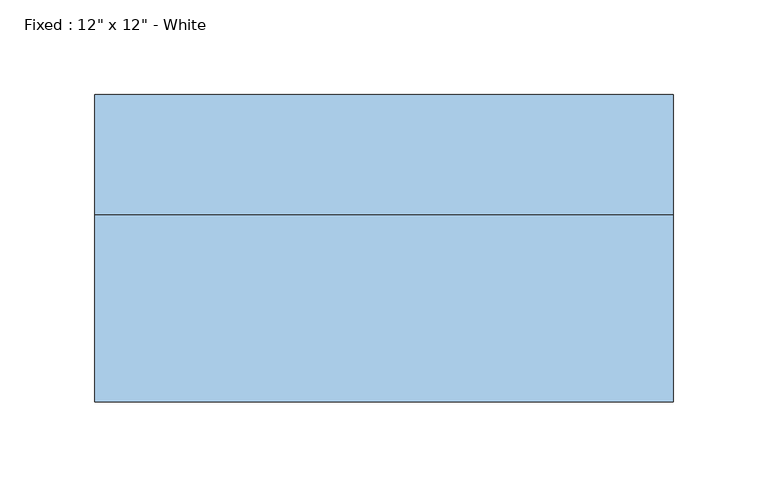
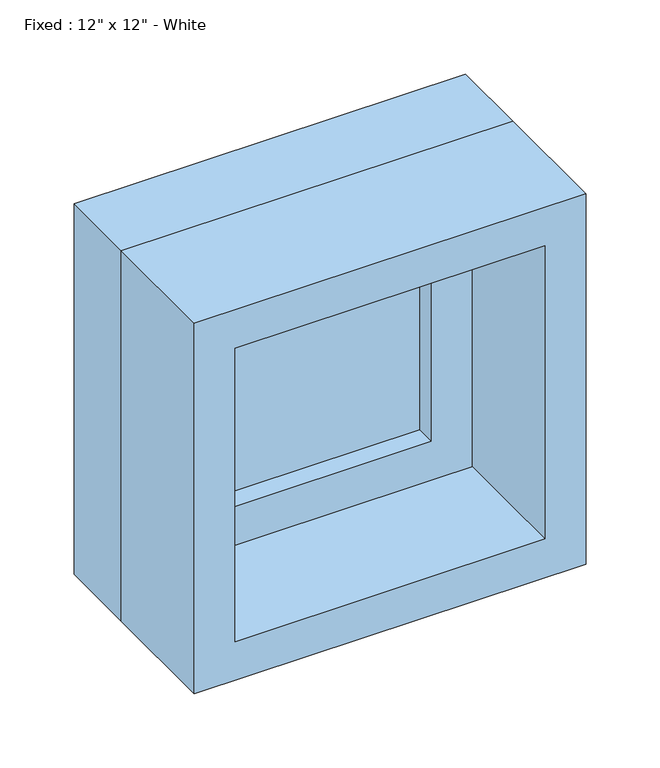
"""IFC4 building model written with IfcOpenShell, lengths in millimetres: window geometry."""

from ifc_helpers import new_model, si_unit, frame, origin, place, context, project, spatial, polyline, outline, extrude, source, transform, mapped, element, save


def window_839e7a6e(model_context):
    return source(origin(), model_context, "Body", "SweptSolid", [
        extrude(outline(polyline([(50.8, 33.3375), (-127.0, 33.3375), (-127.0, 46.0375), (50.8, 46.0375), (50.8, 33.3375)])), frame((0.0, 0.0, 977.9), z_axis=(0.0, 0.0, 1.0), x_axis=(1.0, 0.0, 0.0)), (0.0, 0.0, 1.0), 177.8),
        extrude(outline(polyline([(1200.15, -171.45), (933.45, -171.45), (933.45, 95.25), (1200.15, 95.25), (1200.15, -171.45)]), holes=[polyline([(1155.7, -127.0), (1155.7, 50.8), (977.9, 50.8), (977.9, -127.0), (1155.7, -127.0)])]), frame((0.0, 17.4625, 0.0), z_axis=(0.0, 1.0, 0.0), x_axis=(0.0, 0.0, 1.0)), (0.0, 0.0, 1.0), 44.45),
        extrude(outline(polyline([(1219.2, -190.5), (914.4, -190.5), (914.4, 114.3), (1219.2, 114.3), (1219.2, -190.5)]), holes=[polyline([(1187.45, -158.75), (1187.45, 82.55), (946.15, 82.55), (946.15, -158.75), (1187.45, -158.75)])]), frame((0.0, -80.9625, 0.0), z_axis=(0.0, 1.0, 0.0), x_axis=(0.0, 0.0, 1.0)), (0.0, 0.0, 1.0), 98.425),
        extrude(outline(polyline([(1219.2, 114.3), (1219.2, -190.5), (914.4, -190.5), (914.4, 114.3), (1219.2, 114.3)]), holes=[polyline([(1200.15, 95.25), (933.45, 95.25), (933.45, -171.45), (1200.15, -171.45), (1200.15, 95.25)])]), frame((0.0, 17.4625, 0.0), z_axis=(0.0, 1.0, 0.0), x_axis=(0.0, 0.0, 1.0)), (0.0, 0.0, 1.0), 63.5),
    ])


if __name__ == "__main__":
    model = new_model("IFC4")
    model_context = context("Model", 3, world=origin())
    ifc_project = project(units=[si_unit("LENGTHUNIT", "METRE", prefix="MILLI")], contexts=[model_context])
    site = spatial("IfcSite", under=ifc_project)
    building = spatial("IfcBuilding", under=site)
    placement = place(None, origin())
    window_shape = window_839e7a6e(model_context)
    element("IfcWindow", 1, ObjectType="Fixed : 12\" x 12\" - White", at=placement, inside=building, context=model_context, shape_type="MappedRepresentation", body=[
        mapped(window_shape, transform((0.0, 0.0, 0.0), x_axis=(1.0, 0.0, 0.0), y_axis=(0.0, 1.0, 0.0), z_axis=(0.0, 0.0, 1.0))),
    ])
    save(model, "model.ifc")

# Revit data of these elements
# Type "Fixed : 12\" x 12\" - White"
#   Type Mark = "76"
#   Construction Type Id = "GSP4R"
#   Assembly Code = "B2020100"
#   Analytic Construction = "1/8 in Pilkington single glazing"
#   Visual Light Transmittance = 0.9
#   Solar Heat Gain Coefficient = 0.78
#   Heat Transfer Coefficient (U) = 3.6886 W/(m²·K)
#   Height = 1' - 0"
#   Default Sill Height = 3' - 0"
#   Width = 1' - 0"
#   Window Inset = 0' - 0 3/4"
#   COBie.Type = no
#   Glass Pane Material = Glass
#   Sash Material = Sash - White
#   Wall Closure = (empty or 0)
# Element 1 (IfcWindow, "Fixed : 12\" x 12\" - White")
#   Materials on its faces: "Sash - White", "Glass"
# Materials
#   "Glass": class "Glass", colour RGB 0 128 192, transparency 0.75, Description = "Soda Lime Glass", Cost = 0
#   "Sash - White": class "Wood", colour RGB 255 255 255, transparency 0, Cost = 0
